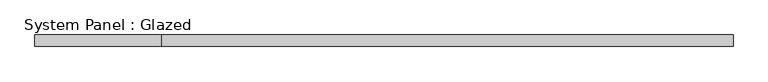
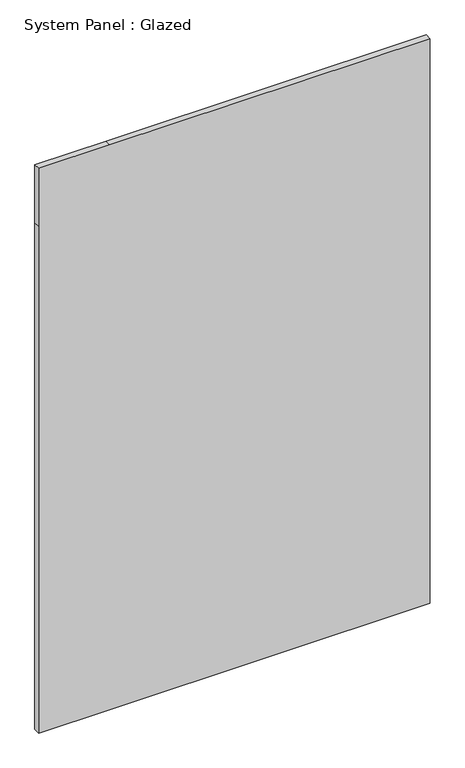
"""IFC4 building model written with IfcOpenShell, lengths in millimetres: plate geometry, System Panel : Glazed."""

import ifcopenshell
import ifcopenshell.guid

model = None  # the IFC model being written
_history = None  # IfcOwnerHistory: only IFC2X3 demands one
_inside = {}  # id of a spatial element -> (the spatial element, [elements in it])
_under = {}  # id of a project, library or spatial element -> (it, [spatial elements below it])
_declared = {}  # id of a project -> (the project, [libraries it declares])
_typed = {}  # id of a type object -> (the type object, [elements of that type])
_made_of = {}  # id of a material, layer set ... -> (it, [elements and type objects made of it])


def new_model(schema):
    """Start an empty IFC model of exactly this schema.

    Asked for "IFC4X3", IfcOpenShell would pick the latest addendum, in which some entities
    have other attributes; the version numbers below select the first issue.
    IFC2X3 requires an IfcOwnerHistory on every rooted entity: one is made here for all.
    """
    global model, _history
    if schema == "IFC4X3":
        model = ifcopenshell.file(schema_version=(4, 3, 0, 0))
    else:
        model = ifcopenshell.file(schema=schema)
    _inside.clear()
    _under.clear()
    _declared.clear()
    _typed.clear()
    _made_of.clear()
    _history = None
    if model.schema == "IFC2X3":
        org = make("IfcOrganization", Name="unknown")
        user = make(
            "IfcPersonAndOrganization",
            ThePerson=make("IfcPerson", FamilyName="unknown"),
            TheOrganization=org,
        )
        app = make(
            "IfcApplication",
            ApplicationDeveloper=org,
            Version="unknown",
            ApplicationFullName="unknown",
            ApplicationIdentifier="unknown",
        )
        _history = make(
            "IfcOwnerHistory",
            OwningUser=user,
            OwningApplication=app,
            ChangeAction="ADDED",
            CreationDate=0,
        )
    return model


def make(cls, **values):
    """One entity of the class cls with the attributes given. An attribute that is None is left unset."""
    return model.create_entity(
        cls, **{name: value for name, value in values.items() if value is not None}
    )


def rooted(cls, **values):
    """An entity with a GlobalId (a new one), such as an element, a storey or a relation."""
    return make(cls, GlobalId=ifcopenshell.guid.new(), OwnerHistory=_history, **values)


def si_unit(unit_type, name, prefix=None):
    """IfcSIUnit, for example si_unit("LENGTHUNIT", "METRE", prefix="MILLI")."""
    return make("IfcSIUnit", UnitType=unit_type, Prefix=prefix, Name=name)


def assignment(units):
    """IfcUnitAssignment: the units of a project."""
    return None if units is None else make("IfcUnitAssignment", Units=units)


def point(xyz):
    """IfcCartesianPoint."""
    return None if xyz is None else make("IfcCartesianPoint", Coordinates=xyz)


def direction(xyz):
    """IfcDirection."""
    return None if xyz is None else make("IfcDirection", DirectionRatios=xyz)


def frame(location, z_axis=None, x_axis=None):
    """IfcAxis2Placement3D, a coordinate frame: its origin and axes. An axis left out is left unset."""
    return make(
        "IfcAxis2Placement3D",
        Location=point(location),
        Axis=direction(z_axis),
        RefDirection=direction(x_axis),
    )


def origin():
    """The frame at (0, 0, 0) with its axes left unset."""
    return frame((0.0, 0.0, 0.0))


def place(relative_to, where):
    """IfcLocalPlacement: puts the frame where relative to a parent placement (None: the world)."""
    return make(
        "IfcLocalPlacement", PlacementRelTo=relative_to, RelativePlacement=where
    )


def context(
    kind, dimensions, precision=None, world=None, true_north=None, identifier=None
):
    """IfcGeometricRepresentationContext, for example the 3D "Model" context."""
    return make(
        "IfcGeometricRepresentationContext",
        ContextIdentifier=identifier,
        ContextType=kind,
        CoordinateSpaceDimension=dimensions,
        Precision=precision,
        WorldCoordinateSystem=world,
        TrueNorth=true_north,
    )


def project(units=None, contexts=None):
    """IfcProject with its units and contexts."""
    return rooted(
        "IfcProject",
        Name="project",
        RepresentationContexts=contexts,
        UnitsInContext=assignment(units),
    )


def spatial(cls, under=None, at=None, **own):
    """A site, building, storey or space (cls), placed at a placement, below another one or the project."""
    s = rooted(cls, ObjectPlacement=at, **own)
    if under is not None:
        _under.setdefault(under.id(), (under, []))[1].append(s)
    return s


def polyline(points):
    """IfcPolyline through the points."""
    return make("IfcPolyline", Points=[point(p) for p in points])


def outline(outer, holes=None, kind="AREA"):
    """IfcArbitraryClosedProfileDef: a profile drawn as a closed curve; with holes, ...WithVoids."""
    if holes is None:
        return make("IfcArbitraryClosedProfileDef", ProfileType=kind, OuterCurve=outer)
    return make(
        "IfcArbitraryProfileDefWithVoids",
        ProfileType=kind,
        OuterCurve=outer,
        InnerCurves=holes,
    )


def extrude(swept, where, along, depth):
    """IfcExtrudedAreaSolid: the profile swept, set in the frame where, extruded along a direction by depth."""
    return make(
        "IfcExtrudedAreaSolid",
        SweptArea=swept,
        Position=where,
        ExtrudedDirection=direction(along),
        Depth=depth,
    )


def shape(context_of_items, identifier, shape_type, items):
    """IfcShapeRepresentation: the items that make up one representation, for example the "Body"."""
    return make(
        "IfcShapeRepresentation",
        ContextOfItems=context_of_items,
        RepresentationIdentifier=identifier,
        RepresentationType=shape_type,
        Items=items,
    )


def source(mapping_origin, context_of_items, identifier, shape_type, items):
    """IfcRepresentationMap: a shape defined once, which mapped items show again and again."""
    return make(
        "IfcRepresentationMap",
        MappingOrigin=mapping_origin,
        MappedRepresentation=shape(context_of_items, identifier, shape_type, items),
    )


def transform(
    local_origin,
    x_axis=None,
    y_axis=None,
    z_axis=None,
    scale=None,
    scale2=None,
    scale3=None,
    uniform=True,
):
    """IfcCartesianTransformationOperator3D, or its non-uniform kind. x_axis, y_axis, z_axis: its Axis1, 2, 3."""
    if uniform:
        return make(
            "IfcCartesianTransformationOperator3D",
            Axis1=direction(x_axis),
            Axis2=direction(y_axis),
            LocalOrigin=point(local_origin),
            Scale=scale,
            Axis3=direction(z_axis),
        )
    return make(
        "IfcCartesianTransformationOperator3DnonUniform",
        Axis1=direction(x_axis),
        Axis2=direction(y_axis),
        LocalOrigin=point(local_origin),
        Scale=scale,
        Axis3=direction(z_axis),
        Scale2=scale2,
        Scale3=scale3,
    )


def mapped(mapping_source, mapping_target):
    """IfcMappedItem: shows the shape of a source again, moved by a transform."""
    return make(
        "IfcMappedItem", MappingSource=mapping_source, MappingTarget=mapping_target
    )


def made_of(thing, what):
    """Note that an element or type object is made of a material, layer set ...; save() writes the relation."""
    if what is not None:
        _made_of.setdefault(what.id(), (what, []))[1].append(thing)
    return thing


def element(
    cls,
    number,
    at=None,
    inside=None,
    cuts=None,
    type_object=None,
    material=None,
    context=None,
    identifier="Body",
    shape_type=None,
    held_by="IfcProductDefinitionShape",
    body=None,
    shapes=None,
    **own,
):
    """One element of the class cls, such as IfcWall. Its Tag is "e" and its number.

    at: its placement. inside: the storey or other place that contains it. cuts: it is an
    opening in that element (IfcRelVoidsElement). A single representation is given by context,
    identifier, shape_type and body (its items); several are given by shapes. held_by: the class
    of the entity that holds the representations. save() writes the other relations.
    """
    e = rooted(cls, Tag="e%d" % number, ObjectPlacement=at, **own)
    if body is not None:
        shapes = [shape(context, identifier, shape_type, body)]
    if shapes is not None:
        e.Representation = make(held_by, Representations=shapes)
    if inside is not None:
        _inside.setdefault(inside.id(), (inside, []))[1].append(e)
    if cuts is not None:
        rooted(
            "IfcRelVoidsElement", RelatingBuildingElement=cuts, RelatedOpeningElement=e
        )
    if type_object is not None:
        _typed.setdefault(type_object.id(), (type_object, []))[1].append(e)
    return made_of(e, material)


def aggregate(whole, parts):
    """IfcRelAggregates: a whole, such as a stair, and the parts it consists of."""
    return rooted("IfcRelAggregates", RelatingObject=whole, RelatedObjects=parts)


def save(model, path):
    """Write the relations noted so far, then the file.

    IfcRelAggregates (storeys below a building ...), IfcRelContainedInSpatialStructure (elements
    in a storey), IfcRelDefinesByType, IfcRelAssociatesMaterial and IfcRelDeclares: one each for
    every whole, place, type object, material and project.
    """
    for whole, parts in _under.values():
        aggregate(whole, parts)
    for where, things in _inside.values():
        rooted(
            "IfcRelContainedInSpatialStructure",
            RelatedElements=things,
            RelatingStructure=where,
        )
    for kind, things in _typed.values():
        rooted("IfcRelDefinesByType", RelatedObjects=things, RelatingType=kind)
    for what, things in _made_of.values():
        rooted("IfcRelAssociatesMaterial", RelatedObjects=things, RelatingMaterial=what)
    for by, libraries in _declared.values():
        rooted("IfcRelDeclares", RelatingContext=by, RelatedDefinitions=libraries)
    model.write(path)


def system_panel_glazed_bb2f95a6(model_context):
    return source(origin(), model_context, "Body", "SweptSolid", [
        extrude(outline(polyline([(0.0, -768.35), (0.0, -488.95), (0.0, 768.35), (2101.85, 768.35), (2343.15, 768.35), (2343.15, -488.95), (2343.15, -768.35), (2101.85, -768.35), (0.0, -768.35)])), frame((0.0, -44.45, 0.0), z_axis=(0.0, 1.0, 0.0), x_axis=(0.0, 0.0, 1.0)), (0.0, 0.0, 1.0), 25.4),
    ])


if __name__ == "__main__":
    model = new_model("IFC4")
    model_context = context("Model", 3, world=origin())
    ifc_project = project(units=[si_unit("LENGTHUNIT", "METRE", prefix="MILLI")], contexts=[model_context])
    site = spatial("IfcSite", under=ifc_project)
    building = spatial("IfcBuilding", under=site)
    placement = place(None, origin())
    system_panel_glazed_shape = system_panel_glazed_bb2f95a6(model_context)
    element("IfcPlate", 1, ObjectType="System Panel : Glazed", at=placement, inside=building, context=model_context, shape_type="MappedRepresentation", body=[
        mapped(system_panel_glazed_shape, transform((0.0, 0.0, 0.0), x_axis=(1.0, 0.0, 0.0), y_axis=(0.0, 1.0, 0.0), z_axis=(0.0, 0.0, 1.0))),
    ])
    save(model, "model.ifc")

# Revit data of these elements
# Element 1 (IfcPlate, "System Panel : Glazed")
#   Materials on its faces: "Glass"
# Materials
#   "Glass": class "Glass", colour RGB 0 128 192, transparency 0.75
